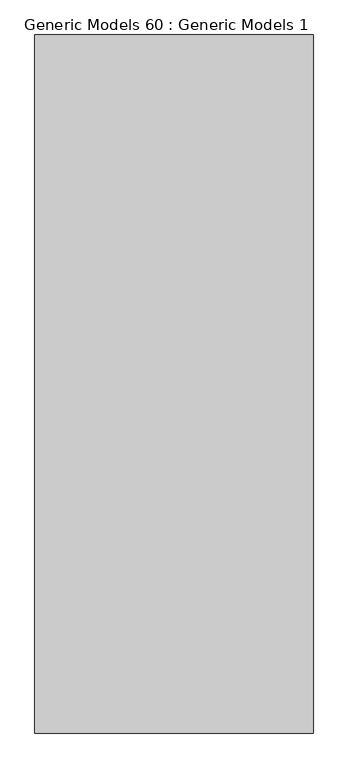
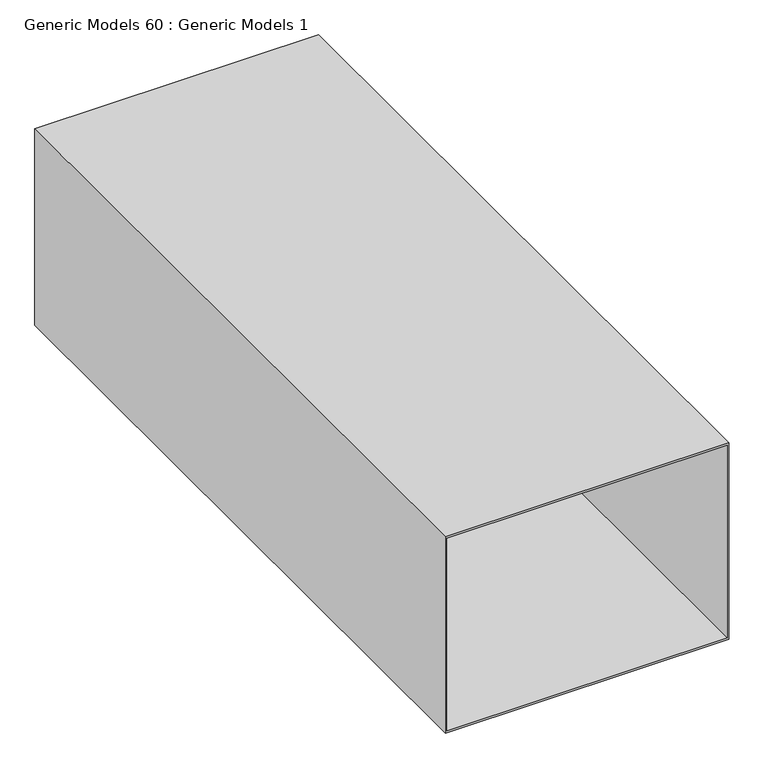
"""IFC4 building model written with IfcOpenShell, lengths in millimetres: proxy geometry, Generic Models 60 : Generic Models 1."""

import ifcopenshell
import ifcopenshell.guid

model = None  # the IFC model being written
_history = None  # IfcOwnerHistory: only IFC2X3 demands one
_inside = {}  # id of a spatial element -> (the spatial element, [elements in it])
_under = {}  # id of a project, library or spatial element -> (it, [spatial elements below it])
_declared = {}  # id of a project -> (the project, [libraries it declares])
_typed = {}  # id of a type object -> (the type object, [elements of that type])
_made_of = {}  # id of a material, layer set ... -> (it, [elements and type objects made of it])


def new_model(schema):
    """Start an empty IFC model of exactly this schema.

    Asked for "IFC4X3", IfcOpenShell would pick the latest addendum, in which some entities
    have other attributes; the version numbers below select the first issue.
    IFC2X3 requires an IfcOwnerHistory on every rooted entity: one is made here for all.
    """
    global model, _history
    if schema == "IFC4X3":
        model = ifcopenshell.file(schema_version=(4, 3, 0, 0))
    else:
        model = ifcopenshell.file(schema=schema)
    _inside.clear()
    _under.clear()
    _declared.clear()
    _typed.clear()
    _made_of.clear()
    _history = None
    if model.schema == "IFC2X3":
        org = make("IfcOrganization", Name="unknown")
        user = make(
            "IfcPersonAndOrganization",
            ThePerson=make("IfcPerson", FamilyName="unknown"),
            TheOrganization=org,
        )
        app = make(
            "IfcApplication",
            ApplicationDeveloper=org,
            Version="unknown",
            ApplicationFullName="unknown",
            ApplicationIdentifier="unknown",
        )
        _history = make(
            "IfcOwnerHistory",
            OwningUser=user,
            OwningApplication=app,
            ChangeAction="ADDED",
            CreationDate=0,
        )
    return model


def make(cls, **values):
    """One entity of the class cls with the attributes given. An attribute that is None is left unset."""
    return model.create_entity(
        cls, **{name: value for name, value in values.items() if value is not None}
    )


def rooted(cls, **values):
    """An entity with a GlobalId (a new one), such as an element, a storey or a relation."""
    return make(cls, GlobalId=ifcopenshell.guid.new(), OwnerHistory=_history, **values)


def si_unit(unit_type, name, prefix=None):
    """IfcSIUnit, for example si_unit("LENGTHUNIT", "METRE", prefix="MILLI")."""
    return make("IfcSIUnit", UnitType=unit_type, Prefix=prefix, Name=name)


def assignment(units):
    """IfcUnitAssignment: the units of a project."""
    return None if units is None else make("IfcUnitAssignment", Units=units)


def point(xyz):
    """IfcCartesianPoint."""
    return None if xyz is None else make("IfcCartesianPoint", Coordinates=xyz)


def direction(xyz):
    """IfcDirection."""
    return None if xyz is None else make("IfcDirection", DirectionRatios=xyz)


def frame(location, z_axis=None, x_axis=None):
    """IfcAxis2Placement3D, a coordinate frame: its origin and axes. An axis left out is left unset."""
    return make(
        "IfcAxis2Placement3D",
        Location=point(location),
        Axis=direction(z_axis),
        RefDirection=direction(x_axis),
    )


def origin():
    """The frame at (0, 0, 0) with its axes left unset."""
    return frame((0.0, 0.0, 0.0))


def place(relative_to, where):
    """IfcLocalPlacement: puts the frame where relative to a parent placement (None: the world)."""
    return make(
        "IfcLocalPlacement", PlacementRelTo=relative_to, RelativePlacement=where
    )


def context(
    kind, dimensions, precision=None, world=None, true_north=None, identifier=None
):
    """IfcGeometricRepresentationContext, for example the 3D "Model" context."""
    return make(
        "IfcGeometricRepresentationContext",
        ContextIdentifier=identifier,
        ContextType=kind,
        CoordinateSpaceDimension=dimensions,
        Precision=precision,
        WorldCoordinateSystem=world,
        TrueNorth=true_north,
    )


def project(units=None, contexts=None):
    """IfcProject with its units and contexts."""
    return rooted(
        "IfcProject",
        Name="project",
        RepresentationContexts=contexts,
        UnitsInContext=assignment(units),
    )


def spatial(cls, under=None, at=None, **own):
    """A site, building, storey or space (cls), placed at a placement, below another one or the project."""
    s = rooted(cls, ObjectPlacement=at, **own)
    if under is not None:
        _under.setdefault(under.id(), (under, []))[1].append(s)
    return s


def polyline(points):
    """IfcPolyline through the points."""
    return make("IfcPolyline", Points=[point(p) for p in points])


def outline(outer, holes=None, kind="AREA"):
    """IfcArbitraryClosedProfileDef: a profile drawn as a closed curve; with holes, ...WithVoids."""
    if holes is None:
        return make("IfcArbitraryClosedProfileDef", ProfileType=kind, OuterCurve=outer)
    return make(
        "IfcArbitraryProfileDefWithVoids",
        ProfileType=kind,
        OuterCurve=outer,
        InnerCurves=holes,
    )


def extrude(swept, where, along, depth):
    """IfcExtrudedAreaSolid: the profile swept, set in the frame where, extruded along a direction by depth."""
    return make(
        "IfcExtrudedAreaSolid",
        SweptArea=swept,
        Position=where,
        ExtrudedDirection=direction(along),
        Depth=depth,
    )


def shape(context_of_items, identifier, shape_type, items):
    """IfcShapeRepresentation: the items that make up one representation, for example the "Body"."""
    return make(
        "IfcShapeRepresentation",
        ContextOfItems=context_of_items,
        RepresentationIdentifier=identifier,
        RepresentationType=shape_type,
        Items=items,
    )


def source(mapping_origin, context_of_items, identifier, shape_type, items):
    """IfcRepresentationMap: a shape defined once, which mapped items show again and again."""
    return make(
        "IfcRepresentationMap",
        MappingOrigin=mapping_origin,
        MappedRepresentation=shape(context_of_items, identifier, shape_type, items),
    )


def transform(
    local_origin,
    x_axis=None,
    y_axis=None,
    z_axis=None,
    scale=None,
    scale2=None,
    scale3=None,
    uniform=True,
):
    """IfcCartesianTransformationOperator3D, or its non-uniform kind. x_axis, y_axis, z_axis: its Axis1, 2, 3."""
    if uniform:
        return make(
            "IfcCartesianTransformationOperator3D",
            Axis1=direction(x_axis),
            Axis2=direction(y_axis),
            LocalOrigin=point(local_origin),
            Scale=scale,
            Axis3=direction(z_axis),
        )
    return make(
        "IfcCartesianTransformationOperator3DnonUniform",
        Axis1=direction(x_axis),
        Axis2=direction(y_axis),
        LocalOrigin=point(local_origin),
        Scale=scale,
        Axis3=direction(z_axis),
        Scale2=scale2,
        Scale3=scale3,
    )


def mapped(mapping_source, mapping_target):
    """IfcMappedItem: shows the shape of a source again, moved by a transform."""
    return make(
        "IfcMappedItem", MappingSource=mapping_source, MappingTarget=mapping_target
    )


def made_of(thing, what):
    """Note that an element or type object is made of a material, layer set ...; save() writes the relation."""
    if what is not None:
        _made_of.setdefault(what.id(), (what, []))[1].append(thing)
    return thing


def element(
    cls,
    number,
    at=None,
    inside=None,
    cuts=None,
    type_object=None,
    material=None,
    context=None,
    identifier="Body",
    shape_type=None,
    held_by="IfcProductDefinitionShape",
    body=None,
    shapes=None,
    **own,
):
    """One element of the class cls, such as IfcWall. Its Tag is "e" and its number.

    at: its placement. inside: the storey or other place that contains it. cuts: it is an
    opening in that element (IfcRelVoidsElement). A single representation is given by context,
    identifier, shape_type and body (its items); several are given by shapes. held_by: the class
    of the entity that holds the representations. save() writes the other relations.
    """
    e = rooted(cls, Tag="e%d" % number, ObjectPlacement=at, **own)
    if body is not None:
        shapes = [shape(context, identifier, shape_type, body)]
    if shapes is not None:
        e.Representation = make(held_by, Representations=shapes)
    if inside is not None:
        _inside.setdefault(inside.id(), (inside, []))[1].append(e)
    if cuts is not None:
        rooted(
            "IfcRelVoidsElement", RelatingBuildingElement=cuts, RelatedOpeningElement=e
        )
    if type_object is not None:
        _typed.setdefault(type_object.id(), (type_object, []))[1].append(e)
    return made_of(e, material)


def aggregate(whole, parts):
    """IfcRelAggregates: a whole, such as a stair, and the parts it consists of."""
    return rooted("IfcRelAggregates", RelatingObject=whole, RelatedObjects=parts)


def save(model, path):
    """Write the relations noted so far, then the file.

    IfcRelAggregates (storeys below a building ...), IfcRelContainedInSpatialStructure (elements
    in a storey), IfcRelDefinesByType, IfcRelAssociatesMaterial and IfcRelDeclares: one each for
    every whole, place, type object, material and project.
    """
    for whole, parts in _under.values():
        aggregate(whole, parts)
    for where, things in _inside.values():
        rooted(
            "IfcRelContainedInSpatialStructure",
            RelatedElements=things,
            RelatingStructure=where,
        )
    for kind, things in _typed.values():
        rooted("IfcRelDefinesByType", RelatedObjects=things, RelatingType=kind)
    for what, things in _made_of.values():
        rooted("IfcRelAssociatesMaterial", RelatedObjects=things, RelatingMaterial=what)
    for by, libraries in _declared.values():
        rooted("IfcRelDeclares", RelatingContext=by, RelatedDefinitions=libraries)
    model.write(path)


def generic_models_60_generic_models_1_d31512ee(model_context):
    return source(origin(), model_context, "Body", "SweptSolid", [
        extrude(outline(polyline([(2028.825, 50664.9319345), (2028.825, 51151.5547769), (2384.425, 51151.5547769), (2384.425, 50664.9319345), (2028.825, 50664.9319345)]), holes=[polyline([(2381.25, 51148.3797769), (2032.0, 51148.3797769), (2032.0, 50668.1069345), (2381.25, 50668.1069345), (2381.25, 51148.3797769)])]), frame((0.0, 0.0, 0.0), z_axis=(0.0, 1.0, 0.0), x_axis=(0.0, 0.0, 1.0)), (0.0, 0.0, 1.0), 1219.2),
    ])


if __name__ == "__main__":
    model = new_model("IFC4")
    model_context = context("Model", 3, world=origin())
    ifc_project = project(units=[si_unit("LENGTHUNIT", "METRE", prefix="MILLI")], contexts=[model_context])
    site = spatial("IfcSite", under=ifc_project)
    building = spatial("IfcBuilding", under=site)
    placement = place(None, origin())
    generic_models_60_generic_models_1_shape = generic_models_60_generic_models_1_d31512ee(model_context)
    element("IfcBuildingElementProxy", 1, Name="Generic Models 60 : Generic Models 1", ObjectType="Generic Models 60 : Generic Models 1", at=placement, inside=building, context=model_context, shape_type="MappedRepresentation", body=[
        mapped(generic_models_60_generic_models_1_shape, transform((0.0, 0.0, 0.0), x_axis=(1.0, 0.0, 0.0), y_axis=(0.0, 1.0, 0.0), z_axis=(0.0, 0.0, 1.0))),
    ])
    save(model, "model.ifc")

# Revit data of these elements
# Element 1 (IfcBuildingElementProxy, "Generic Models 60 : Generic Models 1")
#   Materials on its faces: "EXISTING DUCT"
# Materials
#   "EXISTING DUCT": class "Generic", colour RGB 120 120 120, transparency 0, Cost = 0
